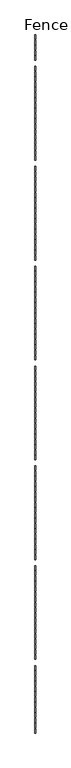
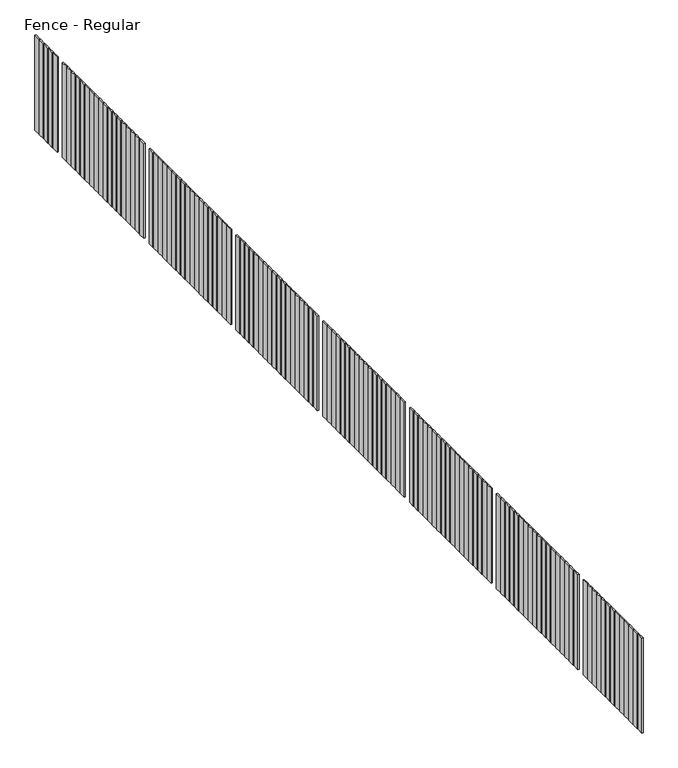
"""IFC4 building model written with IfcOpenShell, lengths in millimetres: railing geometry, Fence - Regular."""

import ifcopenshell
import ifcopenshell.guid

model = None  # the IFC model being written
_history = None  # IfcOwnerHistory: only IFC2X3 demands one
_inside = {}  # id of a spatial element -> (the spatial element, [elements in it])
_under = {}  # id of a project, library or spatial element -> (it, [spatial elements below it])
_declared = {}  # id of a project -> (the project, [libraries it declares])
_typed = {}  # id of a type object -> (the type object, [elements of that type])
_made_of = {}  # id of a material, layer set ... -> (it, [elements and type objects made of it])


def new_model(schema):
    """Start an empty IFC model of exactly this schema.

    Asked for "IFC4X3", IfcOpenShell would pick the latest addendum, in which some entities
    have other attributes; the version numbers below select the first issue.
    IFC2X3 requires an IfcOwnerHistory on every rooted entity: one is made here for all.
    """
    global model, _history
    if schema == "IFC4X3":
        model = ifcopenshell.file(schema_version=(4, 3, 0, 0))
    else:
        model = ifcopenshell.file(schema=schema)
    _inside.clear()
    _under.clear()
    _declared.clear()
    _typed.clear()
    _made_of.clear()
    _history = None
    if model.schema == "IFC2X3":
        org = make("IfcOrganization", Name="unknown")
        user = make(
            "IfcPersonAndOrganization",
            ThePerson=make("IfcPerson", FamilyName="unknown"),
            TheOrganization=org,
        )
        app = make(
            "IfcApplication",
            ApplicationDeveloper=org,
            Version="unknown",
            ApplicationFullName="unknown",
            ApplicationIdentifier="unknown",
        )
        _history = make(
            "IfcOwnerHistory",
            OwningUser=user,
            OwningApplication=app,
            ChangeAction="ADDED",
            CreationDate=0,
        )
    return model


def make(cls, **values):
    """One entity of the class cls with the attributes given. An attribute that is None is left unset."""
    return model.create_entity(
        cls, **{name: value for name, value in values.items() if value is not None}
    )


def rooted(cls, **values):
    """An entity with a GlobalId (a new one), such as an element, a storey or a relation."""
    return make(cls, GlobalId=ifcopenshell.guid.new(), OwnerHistory=_history, **values)


def si_unit(unit_type, name, prefix=None):
    """IfcSIUnit, for example si_unit("LENGTHUNIT", "METRE", prefix="MILLI")."""
    return make("IfcSIUnit", UnitType=unit_type, Prefix=prefix, Name=name)


def assignment(units):
    """IfcUnitAssignment: the units of a project."""
    return None if units is None else make("IfcUnitAssignment", Units=units)


def point(xyz):
    """IfcCartesianPoint."""
    return None if xyz is None else make("IfcCartesianPoint", Coordinates=xyz)


def direction(xyz):
    """IfcDirection."""
    return None if xyz is None else make("IfcDirection", DirectionRatios=xyz)


def frame(location, z_axis=None, x_axis=None):
    """IfcAxis2Placement3D, a coordinate frame: its origin and axes. An axis left out is left unset."""
    return make(
        "IfcAxis2Placement3D",
        Location=point(location),
        Axis=direction(z_axis),
        RefDirection=direction(x_axis),
    )


def origin():
    """The frame at (0, 0, 0) with its axes left unset."""
    return frame((0.0, 0.0, 0.0))


def origin_with_axes():
    """The frame at (0, 0, 0) with the z axis (0, 0, 1) and the x axis (1, 0, 0) written out."""
    return frame((0.0, 0.0, 0.0), z_axis=(0.0, 0.0, 1.0), x_axis=(1.0, 0.0, 0.0))


def place(relative_to, where):
    """IfcLocalPlacement: puts the frame where relative to a parent placement (None: the world)."""
    return make(
        "IfcLocalPlacement", PlacementRelTo=relative_to, RelativePlacement=where
    )


def context(
    kind, dimensions, precision=None, world=None, true_north=None, identifier=None
):
    """IfcGeometricRepresentationContext, for example the 3D "Model" context."""
    return make(
        "IfcGeometricRepresentationContext",
        ContextIdentifier=identifier,
        ContextType=kind,
        CoordinateSpaceDimension=dimensions,
        Precision=precision,
        WorldCoordinateSystem=world,
        TrueNorth=true_north,
    )


def project(units=None, contexts=None):
    """IfcProject with its units and contexts."""
    return rooted(
        "IfcProject",
        Name="project",
        RepresentationContexts=contexts,
        UnitsInContext=assignment(units),
    )


def spatial(cls, under=None, at=None, **own):
    """A site, building, storey or space (cls), placed at a placement, below another one or the project."""
    s = rooted(cls, ObjectPlacement=at, **own)
    if under is not None:
        _under.setdefault(under.id(), (under, []))[1].append(s)
    return s


def polyline(points):
    """IfcPolyline through the points."""
    return make("IfcPolyline", Points=[point(p) for p in points])


def outline(outer, holes=None, kind="AREA"):
    """IfcArbitraryClosedProfileDef: a profile drawn as a closed curve; with holes, ...WithVoids."""
    if holes is None:
        return make("IfcArbitraryClosedProfileDef", ProfileType=kind, OuterCurve=outer)
    return make(
        "IfcArbitraryProfileDefWithVoids",
        ProfileType=kind,
        OuterCurve=outer,
        InnerCurves=holes,
    )


def extrude(swept, where, along, depth):
    """IfcExtrudedAreaSolid: the profile swept, set in the frame where, extruded along a direction by depth."""
    return make(
        "IfcExtrudedAreaSolid",
        SweptArea=swept,
        Position=where,
        ExtrudedDirection=direction(along),
        Depth=depth,
    )


def shape(context_of_items, identifier, shape_type, items):
    """IfcShapeRepresentation: the items that make up one representation, for example the "Body"."""
    return make(
        "IfcShapeRepresentation",
        ContextOfItems=context_of_items,
        RepresentationIdentifier=identifier,
        RepresentationType=shape_type,
        Items=items,
    )


def source(mapping_origin, context_of_items, identifier, shape_type, items):
    """IfcRepresentationMap: a shape defined once, which mapped items show again and again."""
    return make(
        "IfcRepresentationMap",
        MappingOrigin=mapping_origin,
        MappedRepresentation=shape(context_of_items, identifier, shape_type, items),
    )


def transform(
    local_origin,
    x_axis=None,
    y_axis=None,
    z_axis=None,
    scale=None,
    scale2=None,
    scale3=None,
    uniform=True,
):
    """IfcCartesianTransformationOperator3D, or its non-uniform kind. x_axis, y_axis, z_axis: its Axis1, 2, 3."""
    if uniform:
        return make(
            "IfcCartesianTransformationOperator3D",
            Axis1=direction(x_axis),
            Axis2=direction(y_axis),
            LocalOrigin=point(local_origin),
            Scale=scale,
            Axis3=direction(z_axis),
        )
    return make(
        "IfcCartesianTransformationOperator3DnonUniform",
        Axis1=direction(x_axis),
        Axis2=direction(y_axis),
        LocalOrigin=point(local_origin),
        Scale=scale,
        Axis3=direction(z_axis),
        Scale2=scale2,
        Scale3=scale3,
    )


def mapped(mapping_source, mapping_target):
    """IfcMappedItem: shows the shape of a source again, moved by a transform."""
    return make(
        "IfcMappedItem", MappingSource=mapping_source, MappingTarget=mapping_target
    )


def made_of(thing, what):
    """Note that an element or type object is made of a material, layer set ...; save() writes the relation."""
    if what is not None:
        _made_of.setdefault(what.id(), (what, []))[1].append(thing)
    return thing


def element(
    cls,
    number,
    at=None,
    inside=None,
    cuts=None,
    type_object=None,
    material=None,
    context=None,
    identifier="Body",
    shape_type=None,
    held_by="IfcProductDefinitionShape",
    body=None,
    shapes=None,
    **own,
):
    """One element of the class cls, such as IfcWall. Its Tag is "e" and its number.

    at: its placement. inside: the storey or other place that contains it. cuts: it is an
    opening in that element (IfcRelVoidsElement). A single representation is given by context,
    identifier, shape_type and body (its items); several are given by shapes. held_by: the class
    of the entity that holds the representations. save() writes the other relations.
    """
    e = rooted(cls, Tag="e%d" % number, ObjectPlacement=at, **own)
    if body is not None:
        shapes = [shape(context, identifier, shape_type, body)]
    if shapes is not None:
        e.Representation = make(held_by, Representations=shapes)
    if inside is not None:
        _inside.setdefault(inside.id(), (inside, []))[1].append(e)
    if cuts is not None:
        rooted(
            "IfcRelVoidsElement", RelatingBuildingElement=cuts, RelatedOpeningElement=e
        )
    if type_object is not None:
        _typed.setdefault(type_object.id(), (type_object, []))[1].append(e)
    return made_of(e, material)


def aggregate(whole, parts):
    """IfcRelAggregates: a whole, such as a stair, and the parts it consists of."""
    return rooted("IfcRelAggregates", RelatingObject=whole, RelatedObjects=parts)


def save(model, path):
    """Write the relations noted so far, then the file.

    IfcRelAggregates (storeys below a building ...), IfcRelContainedInSpatialStructure (elements
    in a storey), IfcRelDefinesByType, IfcRelAssociatesMaterial and IfcRelDeclares: one each for
    every whole, place, type object, material and project.
    """
    for whole, parts in _under.values():
        aggregate(whole, parts)
    for where, things in _inside.values():
        rooted(
            "IfcRelContainedInSpatialStructure",
            RelatedElements=things,
            RelatingStructure=where,
        )
    for kind, things in _typed.values():
        rooted("IfcRelDefinesByType", RelatedObjects=things, RelatingType=kind)
    for what, things in _made_of.values():
        rooted("IfcRelAssociatesMaterial", RelatedObjects=things, RelatingMaterial=what)
    for by, libraries in _declared.values():
        rooted("IfcRelDeclares", RelatingContext=by, RelatedDefinitions=libraries)
    model.write(path)


def fence_regular_5ff9a863(model_context):
    return source(origin(), model_context, "Body", "SweptSolid", [
        extrude(outline(polyline([(34626.2402986, -30120.4917274), (34626.2402986, -30228.4417274), (34607.1902986, -30228.4417274), (34607.1902986, -30120.4917274), (34626.2402986, -30120.4917274)])), origin_with_axes(), (0.0, 0.0, 1.0), 1625.6),
        extrude(outline(polyline([(34626.2402986, -29992.1548853), (34626.2402986, -30100.1048853), (34607.1902986, -30100.1048853), (34607.1902986, -29992.1548853), (34626.2402986, -29992.1548853)])), origin_with_axes(), (0.0, 0.0, 1.0), 1625.6),
        extrude(outline(polyline([(34626.2402986, -29863.8180432), (34626.2402986, -29971.7680432), (34607.1902986, -29971.7680432), (34607.1902986, -29863.8180432), (34626.2402986, -29863.8180432)])), origin_with_axes(), (0.0, 0.0, 1.0), 1625.6),
        extrude(outline(polyline([(34626.2402986, -29735.4812011), (34626.2402986, -29843.4312011), (34607.1902986, -29843.4312011), (34607.1902986, -29735.4812011), (34626.2402986, -29735.4812011)])), origin_with_axes(), (0.0, 0.0, 1.0), 1625.6),
        extrude(outline(polyline([(34626.2402986, -29607.144359), (34626.2402986, -29715.094359), (34607.1902986, -29715.094359), (34607.1902986, -29607.144359), (34626.2402986, -29607.144359)])), origin_with_axes(), (0.0, 0.0, 1.0), 1625.6),
        extrude(outline(polyline([(34626.2402986, -29478.8075169), (34626.2402986, -29586.7575169), (34607.1902986, -29586.7575169), (34607.1902986, -29478.8075169), (34626.2402986, -29478.8075169)])), origin_with_axes(), (0.0, 0.0, 1.0), 1625.6),
        extrude(outline(polyline([(34626.2402986, -29350.4706748), (34626.2402986, -29458.4206748), (34607.1902986, -29458.4206748), (34607.1902986, -29350.4706748), (34626.2402986, -29350.4706748)])), origin_with_axes(), (0.0, 0.0, 1.0), 1625.6),
        extrude(outline(polyline([(34626.2402986, -29222.1338327), (34626.2402986, -29330.0838327), (34607.1902986, -29330.0838327), (34607.1902986, -29222.1338327), (34626.2402986, -29222.1338327)])), origin_with_axes(), (0.0, 0.0, 1.0), 1625.6),
        extrude(outline(polyline([(34626.2402986, -29093.7969906), (34626.2402986, -29201.7469906), (34607.1902986, -29201.7469906), (34607.1902986, -29093.7969906), (34626.2402986, -29093.7969906)])), origin_with_axes(), (0.0, 0.0, 1.0), 1625.6),
        extrude(outline(polyline([(34626.2402986, -28965.4601485), (34626.2402986, -29073.4101485), (34607.1902986, -29073.4101485), (34607.1902986, -28965.4601485), (34626.2402986, -28965.4601485)])), origin_with_axes(), (0.0, 0.0, 1.0), 1625.6),
        extrude(outline(polyline([(34626.2402986, -28837.1233064), (34626.2402986, -28945.0733064), (34607.1902986, -28945.0733064), (34607.1902986, -28837.1233064), (34626.2402986, -28837.1233064)])), origin_with_axes(), (0.0, 0.0, 1.0), 1625.6),
        extrude(outline(polyline([(34626.2402986, -28708.7864643), (34626.2402986, -28816.7364643), (34607.1902986, -28816.7364643), (34607.1902986, -28708.7864643), (34626.2402986, -28708.7864643)])), origin_with_axes(), (0.0, 0.0, 1.0), 1625.6),
        extrude(outline(polyline([(34626.2402986, -28580.4496222), (34626.2402986, -28688.3996222), (34607.1902986, -28688.3996222), (34607.1902986, -28580.4496222), (34626.2402986, -28580.4496222)])), origin_with_axes(), (0.0, 0.0, 1.0), 1625.6),
        extrude(outline(polyline([(34626.2402986, -28323.7759379), (34626.2402986, -28431.7259379), (34607.1902986, -28431.7259379), (34607.1902986, -28323.7759379), (34626.2402986, -28323.7759379)])), origin_with_axes(), (0.0, 0.0, 1.0), 1625.6),
        extrude(outline(polyline([(34626.2402986, -28195.4390958), (34626.2402986, -28303.3890958), (34607.1902986, -28303.3890958), (34607.1902986, -28195.4390958), (34626.2402986, -28195.4390958)])), origin_with_axes(), (0.0, 0.0, 1.0), 1625.6),
        extrude(outline(polyline([(34626.2402986, -28067.1022537), (34626.2402986, -28175.0522537), (34607.1902986, -28175.0522537), (34607.1902986, -28067.1022537), (34626.2402986, -28067.1022537)])), origin_with_axes(), (0.0, 0.0, 1.0), 1625.6),
        extrude(outline(polyline([(34626.2402986, -27938.7654116), (34626.2402986, -28046.7154116), (34607.1902986, -28046.7154116), (34607.1902986, -27938.7654116), (34626.2402986, -27938.7654116)])), origin_with_axes(), (0.0, 0.0, 1.0), 1625.6),
        extrude(outline(polyline([(34626.2402986, -27810.4285695), (34626.2402986, -27918.3785695), (34607.1902986, -27918.3785695), (34607.1902986, -27810.4285695), (34626.2402986, -27810.4285695)])), origin_with_axes(), (0.0, 0.0, 1.0), 1625.6),
        extrude(outline(polyline([(34626.2402986, -27682.0917274), (34626.2402986, -27790.0417274), (34607.1902986, -27790.0417274), (34607.1902986, -27682.0917274), (34626.2402986, -27682.0917274)])), origin_with_axes(), (0.0, 0.0, 1.0), 1625.6),
        extrude(outline(polyline([(34626.2402986, -27553.7548853), (34626.2402986, -27661.7048853), (34607.1902986, -27661.7048853), (34607.1902986, -27553.7548853), (34626.2402986, -27553.7548853)])), origin_with_axes(), (0.0, 0.0, 1.0), 1625.6),
        extrude(outline(polyline([(34626.2402986, -27425.4180432), (34626.2402986, -27533.3680432), (34607.1902986, -27533.3680432), (34607.1902986, -27425.4180432), (34626.2402986, -27425.4180432)])), origin_with_axes(), (0.0, 0.0, 1.0), 1625.6),
        extrude(outline(polyline([(34626.2402986, -27297.0812011), (34626.2402986, -27405.0312011), (34607.1902986, -27405.0312011), (34607.1902986, -27297.0812011), (34626.2402986, -27297.0812011)])), origin_with_axes(), (0.0, 0.0, 1.0), 1625.6),
        extrude(outline(polyline([(34626.2402986, -27168.744359), (34626.2402986, -27276.694359), (34607.1902986, -27276.694359), (34607.1902986, -27168.744359), (34626.2402986, -27168.744359)])), origin_with_axes(), (0.0, 0.0, 1.0), 1625.6),
        extrude(outline(polyline([(34626.2402986, -27040.4075169), (34626.2402986, -27148.3575169), (34607.1902986, -27148.3575169), (34607.1902986, -27040.4075169), (34626.2402986, -27040.4075169)])), origin_with_axes(), (0.0, 0.0, 1.0), 1625.6),
        extrude(outline(polyline([(34626.2402986, -26912.0706748), (34626.2402986, -27020.0206748), (34607.1902986, -27020.0206748), (34607.1902986, -26912.0706748), (34626.2402986, -26912.0706748)])), origin_with_axes(), (0.0, 0.0, 1.0), 1625.6),
        extrude(outline(polyline([(34626.2402986, -26783.7338327), (34626.2402986, -26891.6838327), (34607.1902986, -26891.6838327), (34607.1902986, -26783.7338327), (34626.2402986, -26783.7338327)])), origin_with_axes(), (0.0, 0.0, 1.0), 1625.6),
        extrude(outline(polyline([(34626.2402986, -26655.3969906), (34626.2402986, -26763.3469906), (34607.1902986, -26763.3469906), (34607.1902986, -26655.3969906), (34626.2402986, -26655.3969906)])), origin_with_axes(), (0.0, 0.0, 1.0), 1625.6),
        extrude(outline(polyline([(34626.2402986, -26527.0601485), (34626.2402986, -26635.0101485), (34607.1902986, -26635.0101485), (34607.1902986, -26527.0601485), (34626.2402986, -26527.0601485)])), origin_with_axes(), (0.0, 0.0, 1.0), 1625.6),
        extrude(outline(polyline([(34626.2402986, -26398.7233064), (34626.2402986, -26506.6733064), (34607.1902986, -26506.6733064), (34607.1902986, -26398.7233064), (34626.2402986, -26398.7233064)])), origin_with_axes(), (0.0, 0.0, 1.0), 1625.6),
        extrude(outline(polyline([(34626.2402986, -26270.3864643), (34626.2402986, -26378.3364643), (34607.1902986, -26378.3364643), (34607.1902986, -26270.3864643), (34626.2402986, -26270.3864643)])), origin_with_axes(), (0.0, 0.0, 1.0), 1625.6),
        extrude(outline(polyline([(34626.2402986, -26142.0496222), (34626.2402986, -26249.9996222), (34607.1902986, -26249.9996222), (34607.1902986, -26142.0496222), (34626.2402986, -26142.0496222)])), origin_with_axes(), (0.0, 0.0, 1.0), 1625.6),
        extrude(outline(polyline([(34626.2402986, -25885.3759379), (34626.2402986, -25993.3259379), (34607.1902986, -25993.3259379), (34607.1902986, -25885.3759379), (34626.2402986, -25885.3759379)])), origin_with_axes(), (0.0, 0.0, 1.0), 1625.6),
        extrude(outline(polyline([(34626.2402986, -25757.0390958), (34626.2402986, -25864.9890958), (34607.1902986, -25864.9890958), (34607.1902986, -25757.0390958), (34626.2402986, -25757.0390958)])), origin_with_axes(), (0.0, 0.0, 1.0), 1625.6),
        extrude(outline(polyline([(34626.2402986, -25628.7022537), (34626.2402986, -25736.6522537), (34607.1902986, -25736.6522537), (34607.1902986, -25628.7022537), (34626.2402986, -25628.7022537)])), origin_with_axes(), (0.0, 0.0, 1.0), 1625.6),
        extrude(outline(polyline([(34626.2402986, -25500.3654116), (34626.2402986, -25608.3154116), (34607.1902986, -25608.3154116), (34607.1902986, -25500.3654116), (34626.2402986, -25500.3654116)])), origin_with_axes(), (0.0, 0.0, 1.0), 1625.6),
        extrude(outline(polyline([(34626.2402986, -25372.0285695), (34626.2402986, -25479.9785695), (34607.1902986, -25479.9785695), (34607.1902986, -25372.0285695), (34626.2402986, -25372.0285695)])), origin_with_axes(), (0.0, 0.0, 1.0), 1625.6),
        extrude(outline(polyline([(34626.2402986, -25243.6917274), (34626.2402986, -25351.6417274), (34607.1902986, -25351.6417274), (34607.1902986, -25243.6917274), (34626.2402986, -25243.6917274)])), origin_with_axes(), (0.0, 0.0, 1.0), 1625.6),
        extrude(outline(polyline([(34626.2402986, -25115.3548853), (34626.2402986, -25223.3048853), (34607.1902986, -25223.3048853), (34607.1902986, -25115.3548853), (34626.2402986, -25115.3548853)])), origin_with_axes(), (0.0, 0.0, 1.0), 1625.6),
        extrude(outline(polyline([(34626.2402986, -24987.0180432), (34626.2402986, -25094.9680432), (34607.1902986, -25094.9680432), (34607.1902986, -24987.0180432), (34626.2402986, -24987.0180432)])), origin_with_axes(), (0.0, 0.0, 1.0), 1625.6),
        extrude(outline(polyline([(34626.2402986, -24858.6812011), (34626.2402986, -24966.6312011), (34607.1902986, -24966.6312011), (34607.1902986, -24858.6812011), (34626.2402986, -24858.6812011)])), origin_with_axes(), (0.0, 0.0, 1.0), 1625.6),
        extrude(outline(polyline([(34626.2402986, -24730.344359), (34626.2402986, -24838.294359), (34607.1902986, -24838.294359), (34607.1902986, -24730.344359), (34626.2402986, -24730.344359)])), origin_with_axes(), (0.0, 0.0, 1.0), 1625.6),
        extrude(outline(polyline([(34626.2402986, -24602.0075169), (34626.2402986, -24709.9575169), (34607.1902986, -24709.9575169), (34607.1902986, -24602.0075169), (34626.2402986, -24602.0075169)])), origin_with_axes(), (0.0, 0.0, 1.0), 1625.6),
        extrude(outline(polyline([(34626.2402986, -24473.6706748), (34626.2402986, -24581.6206748), (34607.1902986, -24581.6206748), (34607.1902986, -24473.6706748), (34626.2402986, -24473.6706748)])), origin_with_axes(), (0.0, 0.0, 1.0), 1625.6),
        extrude(outline(polyline([(34626.2402986, -24345.3338327), (34626.2402986, -24453.2838327), (34607.1902986, -24453.2838327), (34607.1902986, -24345.3338327), (34626.2402986, -24345.3338327)])), origin_with_axes(), (0.0, 0.0, 1.0), 1625.6),
        extrude(outline(polyline([(34626.2402986, -24216.9969906), (34626.2402986, -24324.9469906), (34607.1902986, -24324.9469906), (34607.1902986, -24216.9969906), (34626.2402986, -24216.9969906)])), origin_with_axes(), (0.0, 0.0, 1.0), 1625.6),
        extrude(outline(polyline([(34626.2402986, -24088.6601485), (34626.2402986, -24196.6101485), (34607.1902986, -24196.6101485), (34607.1902986, -24088.6601485), (34626.2402986, -24088.6601485)])), origin_with_axes(), (0.0, 0.0, 1.0), 1625.6),
        extrude(outline(polyline([(34626.2402986, -23960.3233064), (34626.2402986, -24068.2733064), (34607.1902986, -24068.2733064), (34607.1902986, -23960.3233064), (34626.2402986, -23960.3233064)])), origin_with_axes(), (0.0, 0.0, 1.0), 1625.6),
        extrude(outline(polyline([(34626.2402986, -23831.9864643), (34626.2402986, -23939.9364643), (34607.1902986, -23939.9364643), (34607.1902986, -23831.9864643), (34626.2402986, -23831.9864643)])), origin_with_axes(), (0.0, 0.0, 1.0), 1625.6),
        extrude(outline(polyline([(34626.2402986, -23703.6496222), (34626.2402986, -23811.5996222), (34607.1902986, -23811.5996222), (34607.1902986, -23703.6496222), (34626.2402986, -23703.6496222)])), origin_with_axes(), (0.0, 0.0, 1.0), 1625.6),
        extrude(outline(polyline([(34626.2402986, -23446.9759379), (34626.2402986, -23554.9259379), (34607.1902986, -23554.9259379), (34607.1902986, -23446.9759379), (34626.2402986, -23446.9759379)])), origin_with_axes(), (0.0, 0.0, 1.0), 1625.6),
        extrude(outline(polyline([(34626.2402986, -23318.6390958), (34626.2402986, -23426.5890958), (34607.1902986, -23426.5890958), (34607.1902986, -23318.6390958), (34626.2402986, -23318.6390958)])), origin_with_axes(), (0.0, 0.0, 1.0), 1625.6),
        extrude(outline(polyline([(34626.2402986, -23190.3022537), (34626.2402986, -23298.2522537), (34607.1902986, -23298.2522537), (34607.1902986, -23190.3022537), (34626.2402986, -23190.3022537)])), origin_with_axes(), (0.0, 0.0, 1.0), 1625.6),
        extrude(outline(polyline([(34626.2402986, -23061.9654116), (34626.2402986, -23169.9154116), (34607.1902986, -23169.9154116), (34607.1902986, -23061.9654116), (34626.2402986, -23061.9654116)])), origin_with_axes(), (0.0, 0.0, 1.0), 1625.6),
        extrude(outline(polyline([(34626.2402986, -22933.6285695), (34626.2402986, -23041.5785695), (34607.1902986, -23041.5785695), (34607.1902986, -22933.6285695), (34626.2402986, -22933.6285695)])), origin_with_axes(), (0.0, 0.0, 1.0), 1625.6),
        extrude(outline(polyline([(34626.2402986, -22805.2917274), (34626.2402986, -22913.2417274), (34607.1902986, -22913.2417274), (34607.1902986, -22805.2917274), (34626.2402986, -22805.2917274)])), origin_with_axes(), (0.0, 0.0, 1.0), 1625.6),
        extrude(outline(polyline([(34626.2402986, -22676.9548853), (34626.2402986, -22784.9048853), (34607.1902986, -22784.9048853), (34607.1902986, -22676.9548853), (34626.2402986, -22676.9548853)])), origin_with_axes(), (0.0, 0.0, 1.0), 1625.6),
        extrude(outline(polyline([(34626.2402986, -22548.6180432), (34626.2402986, -22656.5680432), (34607.1902986, -22656.5680432), (34607.1902986, -22548.6180432), (34626.2402986, -22548.6180432)])), origin_with_axes(), (0.0, 0.0, 1.0), 1625.6),
        extrude(outline(polyline([(34626.2402986, -22420.2812011), (34626.2402986, -22528.2312011), (34607.1902986, -22528.2312011), (34607.1902986, -22420.2812011), (34626.2402986, -22420.2812011)])), origin_with_axes(), (0.0, 0.0, 1.0), 1625.6),
        extrude(outline(polyline([(34626.2402986, -22291.944359), (34626.2402986, -22399.894359), (34607.1902986, -22399.894359), (34607.1902986, -22291.944359), (34626.2402986, -22291.944359)])), origin_with_axes(), (0.0, 0.0, 1.0), 1625.6),
        extrude(outline(polyline([(34626.2402986, -22163.6075169), (34626.2402986, -22271.5575169), (34607.1902986, -22271.5575169), (34607.1902986, -22163.6075169), (34626.2402986, -22163.6075169)])), origin_with_axes(), (0.0, 0.0, 1.0), 1625.6),
        extrude(outline(polyline([(34626.2402986, -22035.2706748), (34626.2402986, -22143.2206748), (34607.1902986, -22143.2206748), (34607.1902986, -22035.2706748), (34626.2402986, -22035.2706748)])), origin_with_axes(), (0.0, 0.0, 1.0), 1625.6),
        extrude(outline(polyline([(34626.2402986, -21906.9338327), (34626.2402986, -22014.8838327), (34607.1902986, -22014.8838327), (34607.1902986, -21906.9338327), (34626.2402986, -21906.9338327)])), origin_with_axes(), (0.0, 0.0, 1.0), 1625.6),
        extrude(outline(polyline([(34626.2402986, -21778.5969906), (34626.2402986, -21886.5469906), (34607.1902986, -21886.5469906), (34607.1902986, -21778.5969906), (34626.2402986, -21778.5969906)])), origin_with_axes(), (0.0, 0.0, 1.0), 1625.6),
        extrude(outline(polyline([(34626.2402986, -21650.2601485), (34626.2402986, -21758.2101485), (34607.1902986, -21758.2101485), (34607.1902986, -21650.2601485), (34626.2402986, -21650.2601485)])), origin_with_axes(), (0.0, 0.0, 1.0), 1625.6),
        extrude(outline(polyline([(34626.2402986, -21521.9233064), (34626.2402986, -21629.8733064), (34607.1902986, -21629.8733064), (34607.1902986, -21521.9233064), (34626.2402986, -21521.9233064)])), origin_with_axes(), (0.0, 0.0, 1.0), 1625.6),
        extrude(outline(polyline([(34626.2402986, -21393.5864643), (34626.2402986, -21501.5364643), (34607.1902986, -21501.5364643), (34607.1902986, -21393.5864643), (34626.2402986, -21393.5864643)])), origin_with_axes(), (0.0, 0.0, 1.0), 1625.6),
        extrude(outline(polyline([(34626.2402986, -21265.2496222), (34626.2402986, -21373.1996222), (34607.1902986, -21373.1996222), (34607.1902986, -21265.2496222), (34626.2402986, -21265.2496222)])), origin_with_axes(), (0.0, 0.0, 1.0), 1625.6),
        extrude(outline(polyline([(34626.2402986, -21008.5759379), (34626.2402986, -21116.5259379), (34607.1902986, -21116.5259379), (34607.1902986, -21008.5759379), (34626.2402986, -21008.5759379)])), origin_with_axes(), (0.0, 0.0, 1.0), 1625.6),
        extrude(outline(polyline([(34626.2402986, -20880.2390958), (34626.2402986, -20988.1890958), (34607.1902986, -20988.1890958), (34607.1902986, -20880.2390958), (34626.2402986, -20880.2390958)])), origin_with_axes(), (0.0, 0.0, 1.0), 1625.6),
        extrude(outline(polyline([(34626.2402986, -20751.9022537), (34626.2402986, -20859.8522537), (34607.1902986, -20859.8522537), (34607.1902986, -20751.9022537), (34626.2402986, -20751.9022537)])), origin_with_axes(), (0.0, 0.0, 1.0), 1625.6),
        extrude(outline(polyline([(34626.2402986, -20623.5654116), (34626.2402986, -20731.5154116), (34607.1902986, -20731.5154116), (34607.1902986, -20623.5654116), (34626.2402986, -20623.5654116)])), origin_with_axes(), (0.0, 0.0, 1.0), 1625.6),
        extrude(outline(polyline([(34626.2402986, -20495.2285695), (34626.2402986, -20603.1785695), (34607.1902986, -20603.1785695), (34607.1902986, -20495.2285695), (34626.2402986, -20495.2285695)])), origin_with_axes(), (0.0, 0.0, 1.0), 1625.6),
        extrude(outline(polyline([(34626.2402986, -20366.8917274), (34626.2402986, -20474.8417274), (34607.1902986, -20474.8417274), (34607.1902986, -20366.8917274), (34626.2402986, -20366.8917274)])), origin_with_axes(), (0.0, 0.0, 1.0), 1625.6),
        extrude(outline(polyline([(34626.2402986, -20238.5548853), (34626.2402986, -20346.5048853), (34607.1902986, -20346.5048853), (34607.1902986, -20238.5548853), (34626.2402986, -20238.5548853)])), origin_with_axes(), (0.0, 0.0, 1.0), 1625.6),
        extrude(outline(polyline([(34626.2402986, -20110.2180432), (34626.2402986, -20218.1680432), (34607.1902986, -20218.1680432), (34607.1902986, -20110.2180432), (34626.2402986, -20110.2180432)])), origin_with_axes(), (0.0, 0.0, 1.0), 1625.6),
        extrude(outline(polyline([(34626.2402986, -19981.8812011), (34626.2402986, -20089.8312011), (34607.1902986, -20089.8312011), (34607.1902986, -19981.8812011), (34626.2402986, -19981.8812011)])), origin_with_axes(), (0.0, 0.0, 1.0), 1625.6),
        extrude(outline(polyline([(34626.2402986, -19853.544359), (34626.2402986, -19961.494359), (34607.1902986, -19961.494359), (34607.1902986, -19853.544359), (34626.2402986, -19853.544359)])), origin_with_axes(), (0.0, 0.0, 1.0), 1625.6),
        extrude(outline(polyline([(34626.2402986, -19725.2075169), (34626.2402986, -19833.1575169), (34607.1902986, -19833.1575169), (34607.1902986, -19725.2075169), (34626.2402986, -19725.2075169)])), origin_with_axes(), (0.0, 0.0, 1.0), 1625.6),
        extrude(outline(polyline([(34626.2402986, -19596.8706748), (34626.2402986, -19704.8206748), (34607.1902986, -19704.8206748), (34607.1902986, -19596.8706748), (34626.2402986, -19596.8706748)])), origin_with_axes(), (0.0, 0.0, 1.0), 1625.6),
        extrude(outline(polyline([(34626.2402986, -19468.5338327), (34626.2402986, -19576.4838327), (34607.1902986, -19576.4838327), (34607.1902986, -19468.5338327), (34626.2402986, -19468.5338327)])), origin_with_axes(), (0.0, 0.0, 1.0), 1625.6),
        extrude(outline(polyline([(34626.2402986, -19340.1969906), (34626.2402986, -19448.1469906), (34607.1902986, -19448.1469906), (34607.1902986, -19340.1969906), (34626.2402986, -19340.1969906)])), origin_with_axes(), (0.0, 0.0, 1.0), 1625.6),
        extrude(outline(polyline([(34626.2402986, -19211.8601485), (34626.2402986, -19319.8101485), (34607.1902986, -19319.8101485), (34607.1902986, -19211.8601485), (34626.2402986, -19211.8601485)])), origin_with_axes(), (0.0, 0.0, 1.0), 1625.6),
        extrude(outline(polyline([(34626.2402986, -19083.5233064), (34626.2402986, -19191.4733064), (34607.1902986, -19191.4733064), (34607.1902986, -19083.5233064), (34626.2402986, -19083.5233064)])), origin_with_axes(), (0.0, 0.0, 1.0), 1625.6),
        extrude(outline(polyline([(34626.2402986, -18955.1864643), (34626.2402986, -19063.1364643), (34607.1902986, -19063.1364643), (34607.1902986, -18955.1864643), (34626.2402986, -18955.1864643)])), origin_with_axes(), (0.0, 0.0, 1.0), 1625.6),
        extrude(outline(polyline([(34626.2402986, -18826.8496222), (34626.2402986, -18934.7996222), (34607.1902986, -18934.7996222), (34607.1902986, -18826.8496222), (34626.2402986, -18826.8496222)])), origin_with_axes(), (0.0, 0.0, 1.0), 1625.6),
        extrude(outline(polyline([(34626.2402986, -18570.1759379), (34626.2402986, -18678.1259379), (34607.1902986, -18678.1259379), (34607.1902986, -18570.1759379), (34626.2402986, -18570.1759379)])), origin_with_axes(), (0.0, 0.0, 1.0), 1625.6),
        extrude(outline(polyline([(34626.2402986, -18441.8390958), (34626.2402986, -18549.7890958), (34607.1902986, -18549.7890958), (34607.1902986, -18441.8390958), (34626.2402986, -18441.8390958)])), origin_with_axes(), (0.0, 0.0, 1.0), 1625.6),
        extrude(outline(polyline([(34626.2402986, -18313.5022537), (34626.2402986, -18421.4522537), (34607.1902986, -18421.4522537), (34607.1902986, -18313.5022537), (34626.2402986, -18313.5022537)])), origin_with_axes(), (0.0, 0.0, 1.0), 1625.6),
        extrude(outline(polyline([(34626.2402986, -18185.1654116), (34626.2402986, -18293.1154116), (34607.1902986, -18293.1154116), (34607.1902986, -18185.1654116), (34626.2402986, -18185.1654116)])), origin_with_axes(), (0.0, 0.0, 1.0), 1625.6),
        extrude(outline(polyline([(34626.2402986, -18056.8285695), (34626.2402986, -18164.7785695), (34607.1902986, -18164.7785695), (34607.1902986, -18056.8285695), (34626.2402986, -18056.8285695)])), origin_with_axes(), (0.0, 0.0, 1.0), 1625.6),
        extrude(outline(polyline([(34626.2402986, -17928.4917274), (34626.2402986, -18036.4417274), (34607.1902986, -18036.4417274), (34607.1902986, -17928.4917274), (34626.2402986, -17928.4917274)])), origin_with_axes(), (0.0, 0.0, 1.0), 1625.6),
        extrude(outline(polyline([(34626.2402986, -17800.1548853), (34626.2402986, -17908.1048853), (34607.1902986, -17908.1048853), (34607.1902986, -17800.1548853), (34626.2402986, -17800.1548853)])), origin_with_axes(), (0.0, 0.0, 1.0), 1625.6),
        extrude(outline(polyline([(34626.2402986, -17671.8180432), (34626.2402986, -17779.7680432), (34607.1902986, -17779.7680432), (34607.1902986, -17671.8180432), (34626.2402986, -17671.8180432)])), origin_with_axes(), (0.0, 0.0, 1.0), 1625.6),
        extrude(outline(polyline([(34626.2402986, -17543.4812011), (34626.2402986, -17651.4312011), (34607.1902986, -17651.4312011), (34607.1902986, -17543.4812011), (34626.2402986, -17543.4812011)])), origin_with_axes(), (0.0, 0.0, 1.0), 1625.6),
        extrude(outline(polyline([(34626.2402986, -17415.144359), (34626.2402986, -17523.094359), (34607.1902986, -17523.094359), (34607.1902986, -17415.144359), (34626.2402986, -17415.144359)])), origin_with_axes(), (0.0, 0.0, 1.0), 1625.6),
        extrude(outline(polyline([(34626.2402986, -17286.8075169), (34626.2402986, -17394.7575169), (34607.1902986, -17394.7575169), (34607.1902986, -17286.8075169), (34626.2402986, -17286.8075169)])), origin_with_axes(), (0.0, 0.0, 1.0), 1625.6),
        extrude(outline(polyline([(34626.2402986, -17158.4706748), (34626.2402986, -17266.4206748), (34607.1902986, -17266.4206748), (34607.1902986, -17158.4706748), (34626.2402986, -17158.4706748)])), origin_with_axes(), (0.0, 0.0, 1.0), 1625.6),
        extrude(outline(polyline([(34626.2402986, -17030.1338327), (34626.2402986, -17138.0838327), (34607.1902986, -17138.0838327), (34607.1902986, -17030.1338327), (34626.2402986, -17030.1338327)])), origin_with_axes(), (0.0, 0.0, 1.0), 1625.6),
        extrude(outline(polyline([(34626.2402986, -16901.7969906), (34626.2402986, -17009.7469906), (34607.1902986, -17009.7469906), (34607.1902986, -16901.7969906), (34626.2402986, -16901.7969906)])), origin_with_axes(), (0.0, 0.0, 1.0), 1625.6),
        extrude(outline(polyline([(34626.2402986, -16773.4601485), (34626.2402986, -16881.4101485), (34607.1902986, -16881.4101485), (34607.1902986, -16773.4601485), (34626.2402986, -16773.4601485)])), origin_with_axes(), (0.0, 0.0, 1.0), 1625.6),
        extrude(outline(polyline([(34626.2402986, -16645.1233064), (34626.2402986, -16753.0733064), (34607.1902986, -16753.0733064), (34607.1902986, -16645.1233064), (34626.2402986, -16645.1233064)])), origin_with_axes(), (0.0, 0.0, 1.0), 1625.6),
        extrude(outline(polyline([(34626.2402986, -16516.7864643), (34626.2402986, -16624.7364643), (34607.1902986, -16624.7364643), (34607.1902986, -16516.7864643), (34626.2402986, -16516.7864643)])), origin_with_axes(), (0.0, 0.0, 1.0), 1625.6),
        extrude(outline(polyline([(34626.2402986, -16388.4496222), (34626.2402986, -16496.3996222), (34607.1902986, -16496.3996222), (34607.1902986, -16388.4496222), (34626.2402986, -16388.4496222)])), origin_with_axes(), (0.0, 0.0, 1.0), 1625.6),
        extrude(outline(polyline([(34626.2402986, -16131.7759379), (34626.2402986, -16239.7259379), (34607.1902986, -16239.7259379), (34607.1902986, -16131.7759379), (34626.2402986, -16131.7759379)])), origin_with_axes(), (0.0, 0.0, 1.0), 1625.6),
        extrude(outline(polyline([(34626.2402986, -16003.4390958), (34626.2402986, -16111.3890958), (34607.1902986, -16111.3890958), (34607.1902986, -16003.4390958), (34626.2402986, -16003.4390958)])), origin_with_axes(), (0.0, 0.0, 1.0), 1625.6),
        extrude(outline(polyline([(34626.2402986, -15875.1022537), (34626.2402986, -15983.0522537), (34607.1902986, -15983.0522537), (34607.1902986, -15875.1022537), (34626.2402986, -15875.1022537)])), origin_with_axes(), (0.0, 0.0, 1.0), 1625.6),
        extrude(outline(polyline([(34626.2402986, -15746.7654116), (34626.2402986, -15854.7154116), (34607.1902986, -15854.7154116), (34607.1902986, -15746.7654116), (34626.2402986, -15746.7654116)])), origin_with_axes(), (0.0, 0.0, 1.0), 1625.6),
        extrude(outline(polyline([(34626.2402986, -15618.4285695), (34626.2402986, -15726.3785695), (34607.1902986, -15726.3785695), (34607.1902986, -15618.4285695), (34626.2402986, -15618.4285695)])), origin_with_axes(), (0.0, 0.0, 1.0), 1625.6),
        extrude(outline(polyline([(34626.2402986, -15490.0917274), (34626.2402986, -15598.0417274), (34607.1902986, -15598.0417274), (34607.1902986, -15490.0917274), (34626.2402986, -15490.0917274)])), origin_with_axes(), (0.0, 0.0, 1.0), 1625.6),
        extrude(outline(polyline([(34626.2402986, -15361.7548853), (34626.2402986, -15469.7048853), (34607.1902986, -15469.7048853), (34607.1902986, -15361.7548853), (34626.2402986, -15361.7548853)])), origin_with_axes(), (0.0, 0.0, 1.0), 1625.6),
        extrude(outline(polyline([(34626.2402986, -15233.4180432), (34626.2402986, -15341.3680432), (34607.1902986, -15341.3680432), (34607.1902986, -15233.4180432), (34626.2402986, -15233.4180432)])), origin_with_axes(), (0.0, 0.0, 1.0), 1625.6),
        extrude(outline(polyline([(34626.2402986, -15105.0812011), (34626.2402986, -15213.0312011), (34607.1902986, -15213.0312011), (34607.1902986, -15105.0812011), (34626.2402986, -15105.0812011)])), origin_with_axes(), (0.0, 0.0, 1.0), 1625.6),
        extrude(outline(polyline([(34626.2402986, -14976.744359), (34626.2402986, -15084.694359), (34607.1902986, -15084.694359), (34607.1902986, -14976.744359), (34626.2402986, -14976.744359)])), origin_with_axes(), (0.0, 0.0, 1.0), 1625.6),
        extrude(outline(polyline([(34626.2402986, -14848.4075169), (34626.2402986, -14956.3575169), (34607.1902986, -14956.3575169), (34607.1902986, -14848.4075169), (34626.2402986, -14848.4075169)])), origin_with_axes(), (0.0, 0.0, 1.0), 1625.6),
        extrude(outline(polyline([(34626.2402986, -14720.0706748), (34626.2402986, -14828.0206748), (34607.1902986, -14828.0206748), (34607.1902986, -14720.0706748), (34626.2402986, -14720.0706748)])), origin_with_axes(), (0.0, 0.0, 1.0), 1625.6),
        extrude(outline(polyline([(34626.2402986, -14591.7338327), (34626.2402986, -14699.6838327), (34607.1902986, -14699.6838327), (34607.1902986, -14591.7338327), (34626.2402986, -14591.7338327)])), origin_with_axes(), (0.0, 0.0, 1.0), 1625.6),
        extrude(outline(polyline([(34626.2402986, -14463.3969906), (34626.2402986, -14571.3469906), (34607.1902986, -14571.3469906), (34607.1902986, -14463.3969906), (34626.2402986, -14463.3969906)])), origin_with_axes(), (0.0, 0.0, 1.0), 1625.6),
        extrude(outline(polyline([(34626.2402986, -14335.0601485), (34626.2402986, -14443.0101485), (34607.1902986, -14443.0101485), (34607.1902986, -14335.0601485), (34626.2402986, -14335.0601485)])), origin_with_axes(), (0.0, 0.0, 1.0), 1625.6),
        extrude(outline(polyline([(34626.2402986, -14206.7233064), (34626.2402986, -14314.6733064), (34607.1902986, -14314.6733064), (34607.1902986, -14206.7233064), (34626.2402986, -14206.7233064)])), origin_with_axes(), (0.0, 0.0, 1.0), 1625.6),
        extrude(outline(polyline([(34626.2402986, -14078.3864643), (34626.2402986, -14186.3364643), (34607.1902986, -14186.3364643), (34607.1902986, -14078.3864643), (34626.2402986, -14078.3864643)])), origin_with_axes(), (0.0, 0.0, 1.0), 1625.6),
        extrude(outline(polyline([(34626.2402986, -13950.0496222), (34626.2402986, -14057.9996222), (34607.1902986, -14057.9996222), (34607.1902986, -13950.0496222), (34626.2402986, -13950.0496222)])), origin_with_axes(), (0.0, 0.0, 1.0), 1625.6),
        extrude(outline(polyline([(34626.2402986, -13693.3759379), (34626.2402986, -13801.3259379), (34607.1902986, -13801.3259379), (34607.1902986, -13693.3759379), (34626.2402986, -13693.3759379)])), origin_with_axes(), (0.0, 0.0, 1.0), 1625.6),
        extrude(outline(polyline([(34626.2402986, -13565.0390958), (34626.2402986, -13672.9890958), (34607.1902986, -13672.9890958), (34607.1902986, -13565.0390958), (34626.2402986, -13565.0390958)])), origin_with_axes(), (0.0, 0.0, 1.0), 1625.6),
        extrude(outline(polyline([(34626.2402986, -13436.7022537), (34626.2402986, -13544.6522537), (34607.1902986, -13544.6522537), (34607.1902986, -13436.7022537), (34626.2402986, -13436.7022537)])), origin_with_axes(), (0.0, 0.0, 1.0), 1625.6),
        extrude(outline(polyline([(34626.2402986, -13308.3654116), (34626.2402986, -13416.3154116), (34607.1902986, -13416.3154116), (34607.1902986, -13308.3654116), (34626.2402986, -13308.3654116)])), origin_with_axes(), (0.0, 0.0, 1.0), 1625.6),
        extrude(outline(polyline([(34626.2402986, -13180.0285695), (34626.2402986, -13287.9785695), (34607.1902986, -13287.9785695), (34607.1902986, -13180.0285695), (34626.2402986, -13180.0285695)])), origin_with_axes(), (0.0, 0.0, 1.0), 1625.6),
    ])


if __name__ == "__main__":
    model = new_model("IFC4")
    model_context = context("Model", 3, world=origin())
    ifc_project = project(units=[si_unit("LENGTHUNIT", "METRE", prefix="MILLI")], contexts=[model_context])
    site = spatial("IfcSite", under=ifc_project)
    building = spatial("IfcBuilding", under=site)
    placement = place(None, origin())
    fence_regular_shape = fence_regular_5ff9a863(model_context)
    element("IfcRailing", 1, ObjectType="Fence - Regular", at=placement, inside=building, context=model_context, shape_type="MappedRepresentation", body=[
        mapped(fence_regular_shape, transform((0.0, 0.0, 0.0), x_axis=(1.0, 0.0, 0.0), y_axis=(0.0, 1.0, 0.0), z_axis=(0.0, 0.0, 1.0))),
    ])
    save(model, "model.ifc")

# Revit data of these elements
# Element 1 (IfcRailing, "Fence - Regular")
#   Materials on its faces: "6FT HIGH CEDAR PRIVACY FENCE (SEE DETAIL 3A/A500)"
# Materials
#   "6FT HIGH CEDAR PRIVACY FENCE (SEE DETAIL 3A/A500)": class "Wood", colour RGB 146 120 101, transparency 0, Cost = 0
